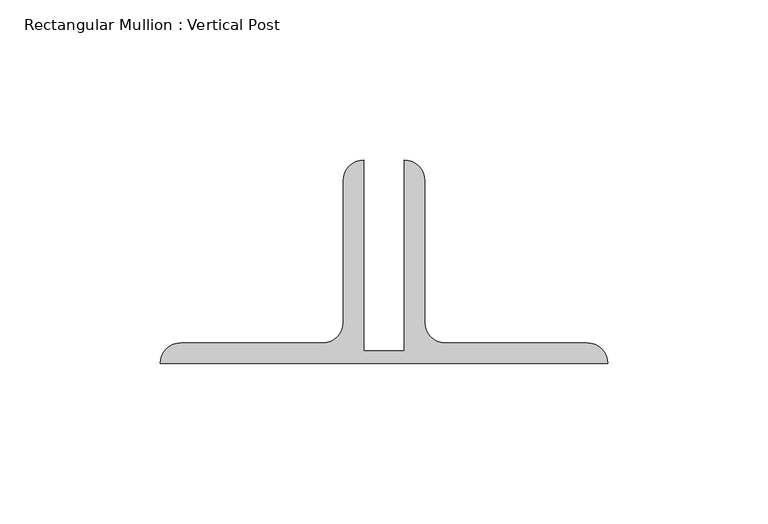
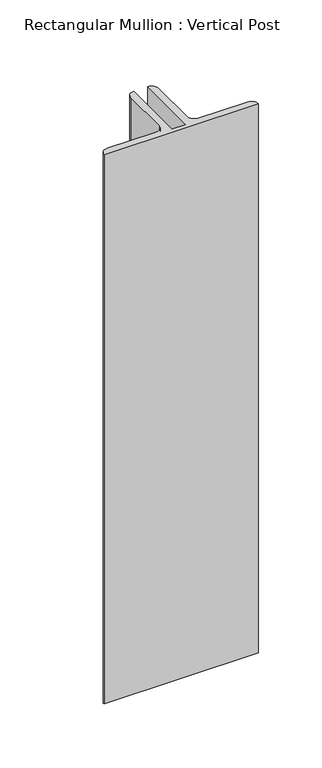
"""IFC4 building model written with IfcOpenShell, lengths in millimetres: member geometry, Rectangular Mullion : Vertical Post."""

from ifc_helpers import new_model, si_unit, point, frame, frame_2d, origin, place, context, project, spatial, polyline, circle_curve, trimmed, segment, composite_curve, outline, extrude, source, transform, mapped, element, save


def rectangular_mullion_vertical_post_b33a09db(model_context):
    return source(origin(), model_context, "Body", "SweptSolid", [
        extrude(outline(composite_curve([segment(polyline([(-76.2, 22.9145205), (-63.5, 22.9145205), (-63.5, 82.55)]), True, "CONTINUOUS"), segment(trimmed(circle_curve(frame_2d((-63.5, 76.2)), 6.35), [point((-63.5, 82.55))], [point((-57.15, 76.2))], False, "CARTESIAN"), True, "CONTINUOUS"), segment(polyline([(-57.15, 76.2), (-57.15, 31.75)]), True, "CONTINUOUS"), segment(trimmed(circle_curve(frame_2d((-50.8, 31.75)), 6.35), [point((-57.15, 31.75))], [point((-50.8, 25.4))], True, "CARTESIAN"), True, "CONTINUOUS"), segment(polyline([(-50.8, 25.4), (-6.35, 25.4)]), True, "CONTINUOUS"), segment(trimmed(circle_curve(frame_2d((-6.35, 19.05)), 6.35), [point((-6.35, 25.4))], [point((0.0, 19.05))], False, "CARTESIAN"), True, "CONTINUOUS"), segment(polyline([(0.0, 19.05), (-139.7, 19.05)]), True, "CONTINUOUS"), segment(trimmed(circle_curve(frame_2d((-133.35, 19.05)), 6.35), [point((-139.7, 19.05))], [point((-133.35, 25.4))], False, "CARTESIAN"), True, "CONTINUOUS"), segment(polyline([(-133.35, 25.4), (-88.9, 25.4)]), True, "CONTINUOUS"), segment(trimmed(circle_curve(frame_2d((-88.9, 31.75)), 6.35), [point((-88.9, 25.4))], [point((-82.55, 31.75))], True, "CARTESIAN"), True, "CONTINUOUS"), segment(polyline([(-82.55, 31.75), (-82.55, 76.2)]), True, "CONTINUOUS"), segment(trimmed(circle_curve(frame_2d((-76.2, 76.2)), 6.35), [point((-82.55, 76.2))], [point((-76.2, 82.55))], False, "CARTESIAN"), True, "CONTINUOUS"), segment(polyline([(-76.2, 82.55), (-76.2, 22.9145205)]), True, "CONTINUOUS")], self_intersect=False)), frame((0.0, 0.0, -526.8889998), z_axis=(0.0, 0.0, 1.0), x_axis=(1.0, 0.0, 0.0)), (0.0, 0.0, 1.0), 526.8889998),
    ])


if __name__ == "__main__":
    model = new_model("IFC4")
    model_context = context("Model", 3, world=origin())
    ifc_project = project(units=[si_unit("LENGTHUNIT", "METRE", prefix="MILLI")], contexts=[model_context])
    site = spatial("IfcSite", under=ifc_project)
    building = spatial("IfcBuilding", under=site)
    placement = place(None, origin())
    rectangular_mullion_vertical_post_shape = rectangular_mullion_vertical_post_b33a09db(model_context)
    element("IfcMember", 1, ObjectType="Rectangular Mullion : Vertical Post", at=placement, inside=building, context=model_context, shape_type="MappedRepresentation", body=[
        mapped(rectangular_mullion_vertical_post_shape, transform((0.0, 0.0, 0.0), x_axis=(1.0, 0.0, 0.0), y_axis=(0.0, 1.0, 0.0), z_axis=(0.0, 0.0, 1.0))),
    ])
    save(model, "model.ifc")

# Revit data of these elements
# Type "Rectangular Mullion : Vertical Post"
#   built-in parameter 1007351 = -0.0625 (stored number, unit not read)
#   built-in parameter 1007322 = 0.0126789 (stored number, unit not read)
#   built-in parameter 1007321 = 0.229167 (stored number, unit not read)
#   built-in parameter 1007320 = 0.229167 (stored number, unit not read)
# Element 1 (IfcMember, "Rectangular Mullion : Vertical Post")
#   Materials on its faces: "GATE POST: (2) BACK/BACK GALVANIZED ANGLES"
# Materials
#   "GATE POST: (2) BACK/BACK GALVANIZED ANGLES": class "Unassigned", colour RGB 211 211 211, transparency 0, Cost = 0
